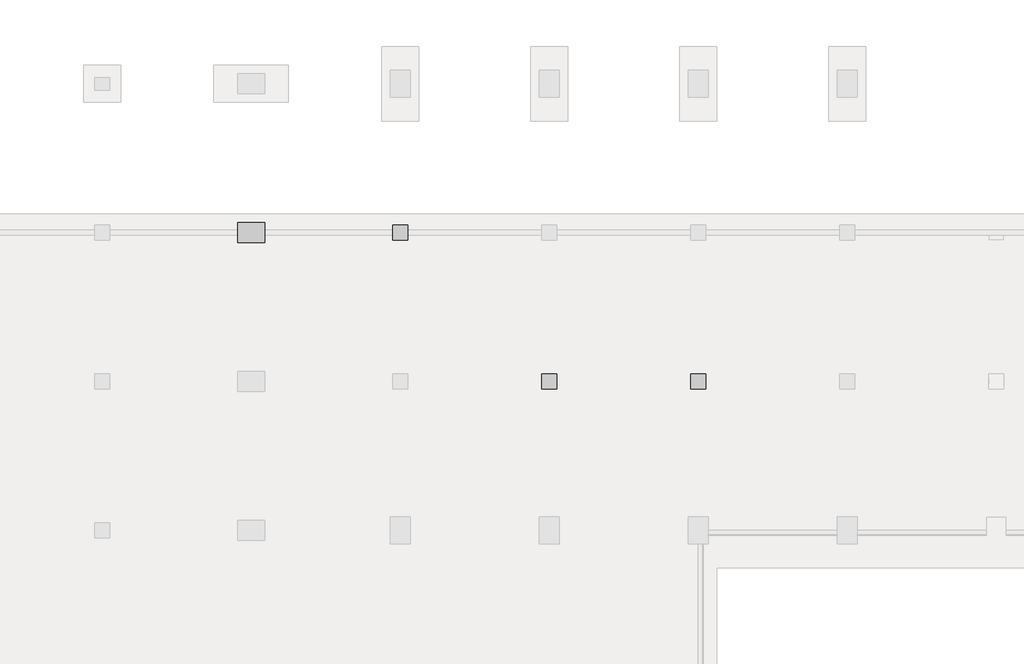
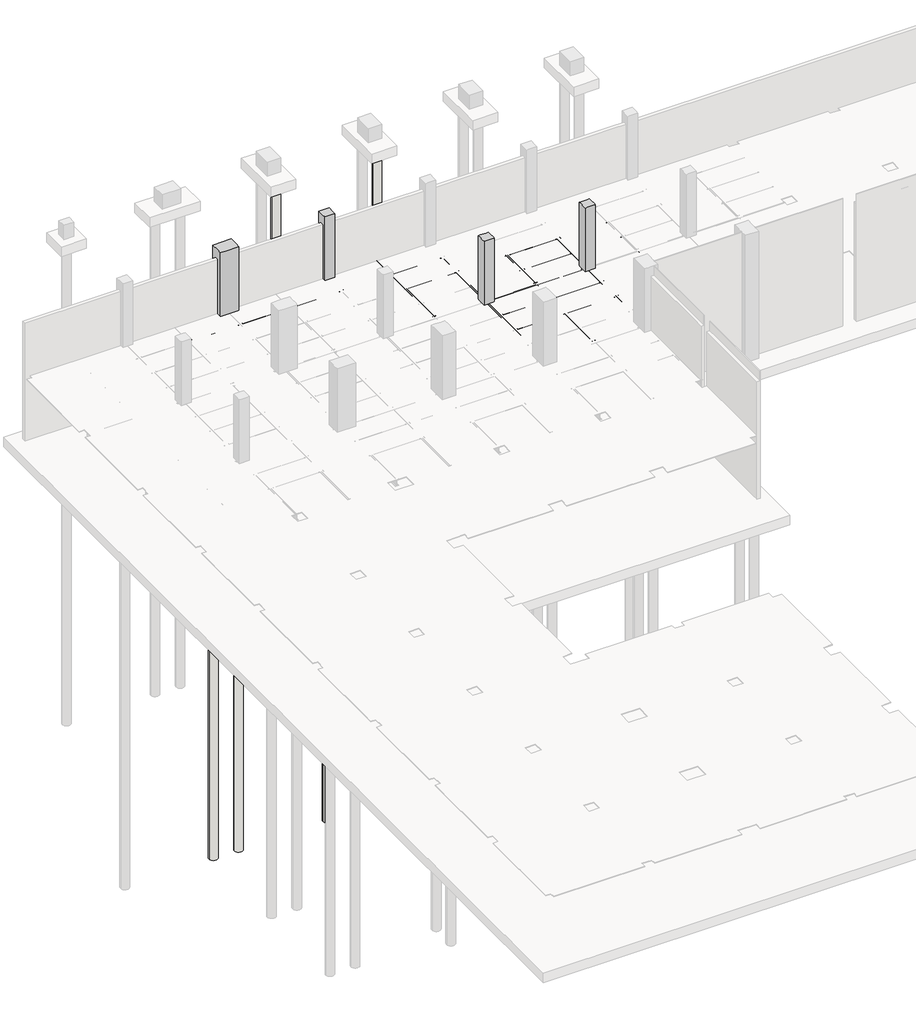
# Not in any storey, part 13 of 16: 29 beams, 6 slabs, 4 columns.
# Revit data of these elements (continued)
# Materials (continued)
#   "Steel, 45-345": class "Metal", colour RGB 189 187 185, transparency 0, Description = "Steel 345 MPa", Cost = 0
#   "00_Concrete_Reinf. Conc.": class "Concrete", colour RGB 176 176 176, transparency 0, Description = "Reinf. Conc.", Cost = 0, Image = Concrete.Cast-In-Place.Flat.Polished.Grey.jpg
#   "Concrete, Precast": class "Concrete", colour RGB 115 116 108, transparency 0, Description = "Precast concrete", Cost = 0
